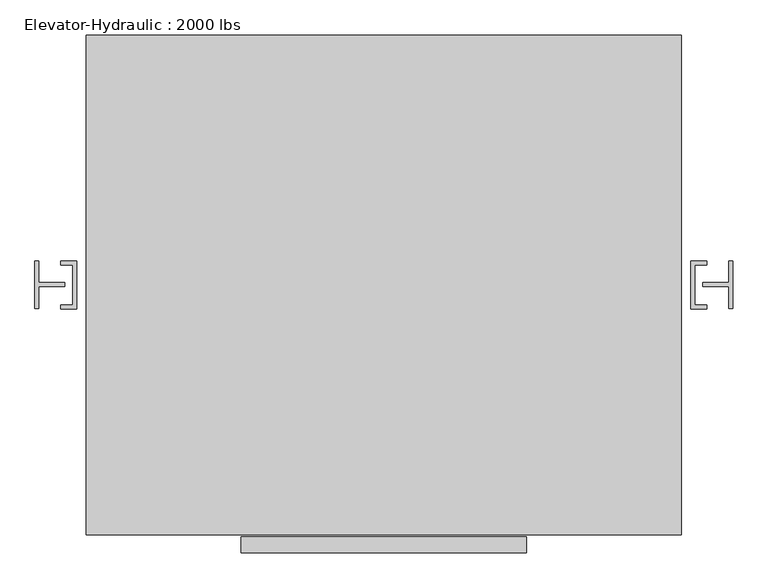
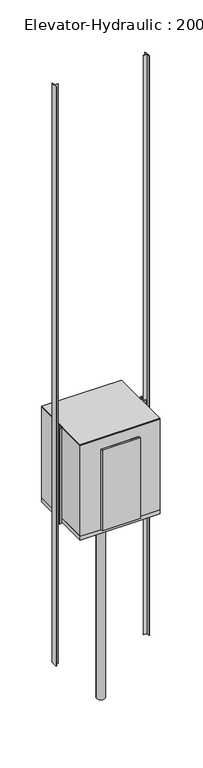
"""IFC4 building model written with IfcOpenShell, lengths in millimetres: proxy geometry, Elevator-Hydraulic : 2000 lbs."""

import ifcopenshell
import ifcopenshell.guid

model = None  # the IFC model being written
_history = None  # IfcOwnerHistory: only IFC2X3 demands one
_inside = {}  # id of a spatial element -> (the spatial element, [elements in it])
_under = {}  # id of a project, library or spatial element -> (it, [spatial elements below it])
_declared = {}  # id of a project -> (the project, [libraries it declares])
_typed = {}  # id of a type object -> (the type object, [elements of that type])
_made_of = {}  # id of a material, layer set ... -> (it, [elements and type objects made of it])


def new_model(schema):
    """Start an empty IFC model of exactly this schema.

    Asked for "IFC4X3", IfcOpenShell would pick the latest addendum, in which some entities
    have other attributes; the version numbers below select the first issue.
    IFC2X3 requires an IfcOwnerHistory on every rooted entity: one is made here for all.
    """
    global model, _history
    if schema == "IFC4X3":
        model = ifcopenshell.file(schema_version=(4, 3, 0, 0))
    else:
        model = ifcopenshell.file(schema=schema)
    _inside.clear()
    _under.clear()
    _declared.clear()
    _typed.clear()
    _made_of.clear()
    _history = None
    if model.schema == "IFC2X3":
        org = make("IfcOrganization", Name="unknown")
        user = make(
            "IfcPersonAndOrganization",
            ThePerson=make("IfcPerson", FamilyName="unknown"),
            TheOrganization=org,
        )
        app = make(
            "IfcApplication",
            ApplicationDeveloper=org,
            Version="unknown",
            ApplicationFullName="unknown",
            ApplicationIdentifier="unknown",
        )
        _history = make(
            "IfcOwnerHistory",
            OwningUser=user,
            OwningApplication=app,
            ChangeAction="ADDED",
            CreationDate=0,
        )
    return model


def make(cls, **values):
    """One entity of the class cls with the attributes given. An attribute that is None is left unset."""
    return model.create_entity(
        cls, **{name: value for name, value in values.items() if value is not None}
    )


def rooted(cls, **values):
    """An entity with a GlobalId (a new one), such as an element, a storey or a relation."""
    return make(cls, GlobalId=ifcopenshell.guid.new(), OwnerHistory=_history, **values)


def si_unit(unit_type, name, prefix=None):
    """IfcSIUnit, for example si_unit("LENGTHUNIT", "METRE", prefix="MILLI")."""
    return make("IfcSIUnit", UnitType=unit_type, Prefix=prefix, Name=name)


def assignment(units):
    """IfcUnitAssignment: the units of a project."""
    return None if units is None else make("IfcUnitAssignment", Units=units)


def point(xyz):
    """IfcCartesianPoint."""
    return None if xyz is None else make("IfcCartesianPoint", Coordinates=xyz)


def direction(xyz):
    """IfcDirection."""
    return None if xyz is None else make("IfcDirection", DirectionRatios=xyz)


def frame(location, z_axis=None, x_axis=None):
    """IfcAxis2Placement3D, a coordinate frame: its origin and axes. An axis left out is left unset."""
    return make(
        "IfcAxis2Placement3D",
        Location=point(location),
        Axis=direction(z_axis),
        RefDirection=direction(x_axis),
    )


def frame_2d(location, x_axis=None):
    """IfcAxis2Placement2D, a coordinate frame in the plane: its origin and x axis."""
    return make(
        "IfcAxis2Placement2D", Location=point(location), RefDirection=direction(x_axis)
    )


def origin():
    """The frame at (0, 0, 0) with its axes left unset."""
    return frame((0.0, 0.0, 0.0))


def origin_with_axes():
    """The frame at (0, 0, 0) with the z axis (0, 0, 1) and the x axis (1, 0, 0) written out."""
    return frame((0.0, 0.0, 0.0), z_axis=(0.0, 0.0, 1.0), x_axis=(1.0, 0.0, 0.0))


def place(relative_to, where):
    """IfcLocalPlacement: puts the frame where relative to a parent placement (None: the world)."""
    return make(
        "IfcLocalPlacement", PlacementRelTo=relative_to, RelativePlacement=where
    )


def context(
    kind, dimensions, precision=None, world=None, true_north=None, identifier=None
):
    """IfcGeometricRepresentationContext, for example the 3D "Model" context."""
    return make(
        "IfcGeometricRepresentationContext",
        ContextIdentifier=identifier,
        ContextType=kind,
        CoordinateSpaceDimension=dimensions,
        Precision=precision,
        WorldCoordinateSystem=world,
        TrueNorth=true_north,
    )


def project(units=None, contexts=None):
    """IfcProject with its units and contexts."""
    return rooted(
        "IfcProject",
        Name="project",
        RepresentationContexts=contexts,
        UnitsInContext=assignment(units),
    )


def spatial(cls, under=None, at=None, **own):
    """A site, building, storey or space (cls), placed at a placement, below another one or the project."""
    s = rooted(cls, ObjectPlacement=at, **own)
    if under is not None:
        _under.setdefault(under.id(), (under, []))[1].append(s)
    return s


def polyline(points):
    """IfcPolyline through the points."""
    return make("IfcPolyline", Points=[point(p) for p in points])


def circle_curve(where, radius):
    """IfcCircle in the frame where."""
    return make("IfcCircle", Position=where, Radius=radius)


def trimmed(basis, trim1, trim2, sense, master):
    """IfcTrimmedCurve: the piece of a basis curve between two trims."""
    return make(
        "IfcTrimmedCurve",
        BasisCurve=basis,
        Trim1=trim1,
        Trim2=trim2,
        SenseAgreement=sense,
        MasterRepresentation=master,
    )


def segment(curve, same_sense, transition):
    """IfcCompositeCurveSegment."""
    return make(
        "IfcCompositeCurveSegment",
        Transition=transition,
        SameSense=same_sense,
        ParentCurve=curve,
    )


def composite_curve(segments, self_intersect=None):
    """IfcCompositeCurve: segments joined end to end."""
    return make("IfcCompositeCurve", Segments=segments, SelfIntersect=self_intersect)


def outline(outer, holes=None, kind="AREA"):
    """IfcArbitraryClosedProfileDef: a profile drawn as a closed curve; with holes, ...WithVoids."""
    if holes is None:
        return make("IfcArbitraryClosedProfileDef", ProfileType=kind, OuterCurve=outer)
    return make(
        "IfcArbitraryProfileDefWithVoids",
        ProfileType=kind,
        OuterCurve=outer,
        InnerCurves=holes,
    )


def extrude(swept, where, along, depth):
    """IfcExtrudedAreaSolid: the profile swept, set in the frame where, extruded along a direction by depth."""
    return make(
        "IfcExtrudedAreaSolid",
        SweptArea=swept,
        Position=where,
        ExtrudedDirection=direction(along),
        Depth=depth,
    )


def faces_of(points, faces, orient=None, outer=None):
    """IfcFace entities. A face is a list of loops; a loop is a list of indices into points, from 0.

    orient and outer hold one flag for each loop. By default every Orientation is true, the
    first loop of a face is its IfcFaceOuterBound and the others are IfcFaceBound.
    """
    made = []
    for i, loops in enumerate(faces):
        bounds = []
        for j, loop in enumerate(loops):
            is_outer = j == 0 if outer is None else outer[i][j]
            bounds.append(
                make(
                    "IfcFaceOuterBound" if is_outer else "IfcFaceBound",
                    Bound=make("IfcPolyLoop", Polygon=[points[k] for k in loop]),
                    Orientation=True if orient is None else orient[i][j],
                )
            )
        made.append(make("IfcFace", Bounds=bounds))
    return made


def faceted_brep(points, faces, orient=None, outer=None, voids=None):
    """IfcFacetedBrep: a solid bounded by flat faces; with voids (closed shells), ...WithVoids."""
    shared = [point(p) for p in points]
    hull = make("IfcClosedShell", CfsFaces=faces_of(shared, faces, orient, outer))
    if voids is None:
        return make("IfcFacetedBrep", Outer=hull)
    return make(
        "IfcFacetedBrepWithVoids",
        Outer=hull,
        Voids=[
            make(cls, CfsFaces=faces_of(shared, fs, o, b)) for cls, fs, o, b in voids
        ],
    )


def shape(context_of_items, identifier, shape_type, items):
    """IfcShapeRepresentation: the items that make up one representation, for example the "Body"."""
    return make(
        "IfcShapeRepresentation",
        ContextOfItems=context_of_items,
        RepresentationIdentifier=identifier,
        RepresentationType=shape_type,
        Items=items,
    )


def source(mapping_origin, context_of_items, identifier, shape_type, items):
    """IfcRepresentationMap: a shape defined once, which mapped items show again and again."""
    return make(
        "IfcRepresentationMap",
        MappingOrigin=mapping_origin,
        MappedRepresentation=shape(context_of_items, identifier, shape_type, items),
    )


def transform(
    local_origin,
    x_axis=None,
    y_axis=None,
    z_axis=None,
    scale=None,
    scale2=None,
    scale3=None,
    uniform=True,
):
    """IfcCartesianTransformationOperator3D, or its non-uniform kind. x_axis, y_axis, z_axis: its Axis1, 2, 3."""
    if uniform:
        return make(
            "IfcCartesianTransformationOperator3D",
            Axis1=direction(x_axis),
            Axis2=direction(y_axis),
            LocalOrigin=point(local_origin),
            Scale=scale,
            Axis3=direction(z_axis),
        )
    return make(
        "IfcCartesianTransformationOperator3DnonUniform",
        Axis1=direction(x_axis),
        Axis2=direction(y_axis),
        LocalOrigin=point(local_origin),
        Scale=scale,
        Axis3=direction(z_axis),
        Scale2=scale2,
        Scale3=scale3,
    )


def mapped(mapping_source, mapping_target):
    """IfcMappedItem: shows the shape of a source again, moved by a transform."""
    return make(
        "IfcMappedItem", MappingSource=mapping_source, MappingTarget=mapping_target
    )


def made_of(thing, what):
    """Note that an element or type object is made of a material, layer set ...; save() writes the relation."""
    if what is not None:
        _made_of.setdefault(what.id(), (what, []))[1].append(thing)
    return thing


def element(
    cls,
    number,
    at=None,
    inside=None,
    cuts=None,
    type_object=None,
    material=None,
    context=None,
    identifier="Body",
    shape_type=None,
    held_by="IfcProductDefinitionShape",
    body=None,
    shapes=None,
    **own,
):
    """One element of the class cls, such as IfcWall. Its Tag is "e" and its number.

    at: its placement. inside: the storey or other place that contains it. cuts: it is an
    opening in that element (IfcRelVoidsElement). A single representation is given by context,
    identifier, shape_type and body (its items); several are given by shapes. held_by: the class
    of the entity that holds the representations. save() writes the other relations.
    """
    e = rooted(cls, Tag="e%d" % number, ObjectPlacement=at, **own)
    if body is not None:
        shapes = [shape(context, identifier, shape_type, body)]
    if shapes is not None:
        e.Representation = make(held_by, Representations=shapes)
    if inside is not None:
        _inside.setdefault(inside.id(), (inside, []))[1].append(e)
    if cuts is not None:
        rooted(
            "IfcRelVoidsElement", RelatingBuildingElement=cuts, RelatedOpeningElement=e
        )
    if type_object is not None:
        _typed.setdefault(type_object.id(), (type_object, []))[1].append(e)
    return made_of(e, material)


def aggregate(whole, parts):
    """IfcRelAggregates: a whole, such as a stair, and the parts it consists of."""
    return rooted("IfcRelAggregates", RelatingObject=whole, RelatedObjects=parts)


def save(model, path):
    """Write the relations noted so far, then the file.

    IfcRelAggregates (storeys below a building ...), IfcRelContainedInSpatialStructure (elements
    in a storey), IfcRelDefinesByType, IfcRelAssociatesMaterial and IfcRelDeclares: one each for
    every whole, place, type object, material and project.
    """
    for whole, parts in _under.values():
        aggregate(whole, parts)
    for where, things in _inside.values():
        rooted(
            "IfcRelContainedInSpatialStructure",
            RelatedElements=things,
            RelatingStructure=where,
        )
    for kind, things in _typed.values():
        rooted("IfcRelDefinesByType", RelatedObjects=things, RelatingType=kind)
    for what, things in _made_of.values():
        rooted("IfcRelAssociatesMaterial", RelatedObjects=things, RelatingMaterial=what)
    for by, libraries in _declared.values():
        rooted("IfcRelDeclares", RelatingContext=by, RelatedDefinitions=libraries)
    model.write(path)


def elevator_hydraulic_2000_lbs_23fd6a1c(model_context):
    return source(origin(), model_context, "Body", "SolidModel", [
        faceted_brep([(-945.0530035, -797.2781737, 5943.6), (959.9469965, -797.2781737, 5943.6), (959.9469965, 802.9218263, 5943.6), (-945.0530035, 802.9218263, 5943.6), (921.8469965, 764.8218263, 5943.6), (921.8469965, -759.1781737, 5943.6), (-906.9530035, -759.1781737, 5943.6), (-906.9530035, 764.8218263, 5943.6), (-906.9530035, 764.8218263, 3657.6), (-906.9530035, -759.1781737, 3657.6), (-449.7530035, -759.1781737, 3657.6), (-449.7530035, -797.2781737, 3657.6), (-945.0530035, -797.2781737, 3657.6), (-945.0530035, 802.9218263, 3657.6), (959.9469965, 802.9218263, 3657.6), (959.9469965, -797.2781737, 3657.6), (464.6469965, -797.2781737, 3657.6), (464.6469965, -759.1781737, 3657.6), (921.8469965, -759.1781737, 3657.6), (921.8469965, 764.8218263, 3657.6), (464.6469965, 764.8218263, 3657.6), (-449.7530035, 764.8218263, 3657.6), (464.6469965, -759.1781737, 5689.6), (-449.7530035, -759.1781737, 5689.6), (-449.7530035, -797.2781737, 5689.6), (464.6469965, -797.2781737, 5689.6)], [[[0, 1, 2, 3], [4, 5, 6, 7]], [[8, 9, 10, 11, 12, 13, 14, 15, 16, 17, 18, 19, 20, 21]], [[5, 4, 19, 18]], [[6, 5, 18, 17, 22, 23, 10, 9]], [[7, 6, 9, 8]], [[4, 7, 8, 21, 20, 19]], [[1, 0, 12, 11, 24, 25, 16, 15]], [[2, 1, 15, 14]], [[3, 2, 14, 13]], [[0, 3, 13, 12]], [[22, 25, 24, 23]], [[23, 24, 11, 10]], [[25, 22, 17, 16]]]),
        extrude(outline(polyline([(464.6469965, -803.6281737), (464.6469965, -854.4281737), (-449.7530035, -854.4281737), (-449.7530035, -803.6281737), (464.6469965, -803.6281737)])), frame((0.0, 0.0, 3657.6), z_axis=(0.0, 0.0, 1.0), x_axis=(1.0, 0.0, 0.0)), (0.0, 0.0, 1.0), 2032.0),
        extrude(outline(polyline([(959.9469965, 802.9218263), (959.9469965, -797.2781737), (-945.0530035, -797.2781737), (-945.0530035, 802.9218263), (959.9469965, 802.9218263)])), frame((0.0, 0.0, 5943.6), z_axis=(0.0, 0.0, 1.0), x_axis=(1.0, 0.0, 0.0)), (0.0, 0.0, 1.0), 25.4),
        extrude(outline(composite_curve([segment(trimmed(circle_curve(frame_2d((7.4469965, 2.8218263)), 101.6), [point((-94.1530035, 2.8218263))], [point((109.0469965, 2.8218263))], False, "CARTESIAN"), True, "CONTINUOUS"), segment(trimmed(circle_curve(frame_2d((7.4469965, 2.8218263)), 101.6), [point((109.0469965, 2.8218263))], [point((-94.1530035, 2.8218263))], False, "CARTESIAN"), True, "CONTINUOUS")], self_intersect=False)), frame((0.0, 0.0, -1219.2), z_axis=(0.0, 0.0, 1.0), x_axis=(1.0, 0.0, 0.0)), (0.0, 0.0, 1.0), 4775.2),
        extrude(outline(polyline([(959.9469965, 802.9218263), (959.9469965, -797.2781737), (-945.0530035, -797.2781737), (-945.0530035, 802.9218263), (959.9469965, 802.9218263)])), frame((0.0, 0.0, 3556.0), z_axis=(0.0, 0.0, 1.0), x_axis=(1.0, 0.0, 0.0)), (0.0, 0.0, 1.0), 101.6),
        extrude(outline(polyline([(-976.8030035, 79.0218263), (-976.8030035, -73.3781737), (-1027.6030035, -73.3781737), (-1027.6030035, -60.6781737), (-989.5030035, -60.6781737), (-989.5030035, 66.3218263), (-1027.6030035, 66.3218263), (-1027.6030035, 79.0218263), (-976.8030035, 79.0218263)])), frame((0.0, 0.0, 3556.0), z_axis=(0.0, 0.0, 1.0), x_axis=(1.0, 0.0, 0.0)), (0.0, 0.0, 1.0), 2413.0),
        extrude(outline(polyline([(991.6969965, 79.0218263), (1042.4969965, 79.0218263), (1042.4969965, 66.3218263), (1004.3969965, 66.3218263), (1004.3969965, -60.6781737), (1042.4969965, -60.6781737), (1042.4969965, -73.3781737), (991.6969965, -73.3781737), (991.6969965, 79.0218263)])), frame((0.0, 0.0, 3556.0), z_axis=(0.0, 0.0, 1.0), x_axis=(1.0, 0.0, 0.0)), (0.0, 0.0, 1.0), 2413.0),
        extrude(outline(polyline([(-1097.4530035, 79.0218263), (-1097.4530035, 9.1718263), (-1014.9030035, 9.1718263), (-1014.9030035, -3.5281737), (-1097.4530035, -3.5281737), (-1097.4530035, -73.3781737), (-1110.1530035, -73.3781737), (-1110.1530035, 79.0218263), (-1097.4530035, 79.0218263)])), origin_with_axes(), (0.0, 0.0, 1.0), 14630.4),
        extrude(outline(polyline([(1112.3469965, 79.0218263), (1125.0469965, 79.0218263), (1125.0469965, -73.3781737), (1112.3469965, -73.3781737), (1112.3469965, -3.5281737), (1029.7969965, -3.5281737), (1029.7969965, 9.1718263), (1112.3469965, 9.1718263), (1112.3469965, 79.0218263)])), origin_with_axes(), (0.0, 0.0, 1.0), 14630.4),
    ])


if __name__ == "__main__":
    model = new_model("IFC4")
    model_context = context("Model", 3, world=origin())
    ifc_project = project(units=[si_unit("LENGTHUNIT", "METRE", prefix="MILLI")], contexts=[model_context])
    site = spatial("IfcSite", under=ifc_project)
    building = spatial("IfcBuilding", under=site)
    placement = place(None, origin())
    elevator_hydraulic_2000_lbs_shape = elevator_hydraulic_2000_lbs_23fd6a1c(model_context)
    element("IfcBuildingElementProxy", 1, Name="Elevator-Hydraulic : 2000 lbs", ObjectType="Elevator-Hydraulic : 2000 lbs", at=placement, inside=building, context=model_context, shape_type="MappedRepresentation", body=[
        mapped(elevator_hydraulic_2000_lbs_shape, transform((0.0, 0.0, 0.0), x_axis=(1.0, 0.0, 0.0), y_axis=(0.0, 1.0, 0.0), z_axis=(0.0, 0.0, 1.0))),
    ])
    save(model, "model.ifc")

# Revit data of these elements
# Type "Elevator-Hydraulic : 2000 lbs"
#   Cab Location = 12' - 0"
#   Width = 7' - 4"
#   Pit Depth = 4' - 0"
#   Height [instance default] = 36' - 0"
#   Door Opening = 3' - 0"
#   Depth = 5' - 9"
#   Cab Width = 6' - 0"
#   Cab Height = 7' - 6"
#   Cab Depth = 5' - 0"
#   Default Elevation = 0
# Element 1 (IfcBuildingElementProxy, "Elevator-Hydraulic : 2000 lbs")
#   Height = 48' - 0"
#   Materials on its faces: "Metal - Steel"
# Materials
#   "Metal - Steel": class "Metal", colour RGB 247 247 247, transparency 0
